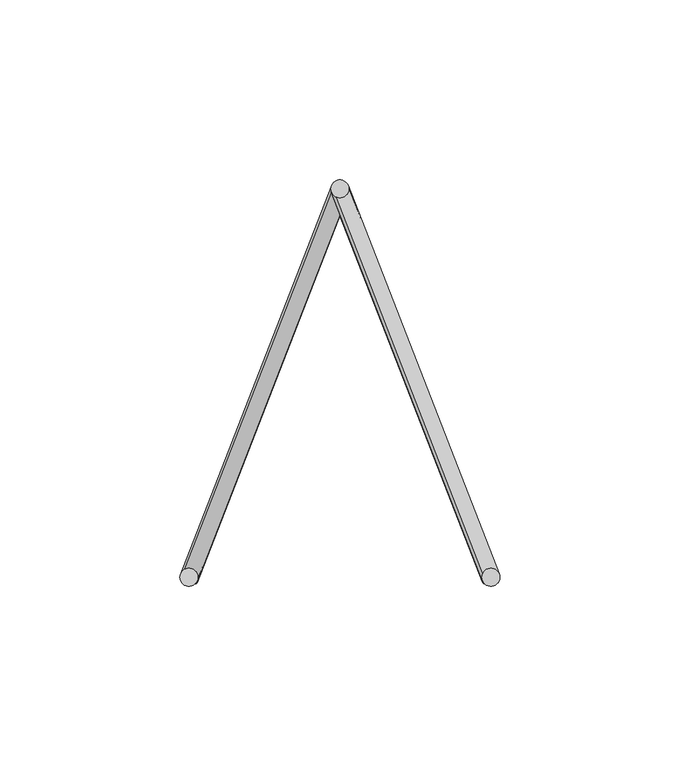
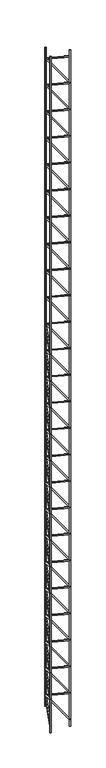
"""IFC4 building model written with IfcOpenShell, lengths in millimetres: proxy geometry, Pre-fab. (Vigota 7 - Pano 3)."""

import ifcopenshell
import ifcopenshell.guid

model = None  # the IFC model being written
_history = None  # IfcOwnerHistory: only IFC2X3 demands one
_inside = {}  # id of a spatial element -> (the spatial element, [elements in it])
_under = {}  # id of a project, library or spatial element -> (it, [spatial elements below it])
_declared = {}  # id of a project -> (the project, [libraries it declares])
_typed = {}  # id of a type object -> (the type object, [elements of that type])
_made_of = {}  # id of a material, layer set ... -> (it, [elements and type objects made of it])


def new_model(schema):
    """Start an empty IFC model of exactly this schema.

    Asked for "IFC4X3", IfcOpenShell would pick the latest addendum, in which some entities
    have other attributes; the version numbers below select the first issue.
    IFC2X3 requires an IfcOwnerHistory on every rooted entity: one is made here for all.
    """
    global model, _history
    if schema == "IFC4X3":
        model = ifcopenshell.file(schema_version=(4, 3, 0, 0))
    else:
        model = ifcopenshell.file(schema=schema)
    _inside.clear()
    _under.clear()
    _declared.clear()
    _typed.clear()
    _made_of.clear()
    _history = None
    if model.schema == "IFC2X3":
        org = make("IfcOrganization", Name="unknown")
        user = make(
            "IfcPersonAndOrganization",
            ThePerson=make("IfcPerson", FamilyName="unknown"),
            TheOrganization=org,
        )
        app = make(
            "IfcApplication",
            ApplicationDeveloper=org,
            Version="unknown",
            ApplicationFullName="unknown",
            ApplicationIdentifier="unknown",
        )
        _history = make(
            "IfcOwnerHistory",
            OwningUser=user,
            OwningApplication=app,
            ChangeAction="ADDED",
            CreationDate=0,
        )
    return model


def make(cls, **values):
    """One entity of the class cls with the attributes given. An attribute that is None is left unset."""
    return model.create_entity(
        cls, **{name: value for name, value in values.items() if value is not None}
    )


def rooted(cls, **values):
    """An entity with a GlobalId (a new one), such as an element, a storey or a relation."""
    return make(cls, GlobalId=ifcopenshell.guid.new(), OwnerHistory=_history, **values)


def si_unit(unit_type, name, prefix=None):
    """IfcSIUnit, for example si_unit("LENGTHUNIT", "METRE", prefix="MILLI")."""
    return make("IfcSIUnit", UnitType=unit_type, Prefix=prefix, Name=name)


def assignment(units):
    """IfcUnitAssignment: the units of a project."""
    return None if units is None else make("IfcUnitAssignment", Units=units)


def point(xyz):
    """IfcCartesianPoint."""
    return None if xyz is None else make("IfcCartesianPoint", Coordinates=xyz)


def direction(xyz):
    """IfcDirection."""
    return None if xyz is None else make("IfcDirection", DirectionRatios=xyz)


def frame(location, z_axis=None, x_axis=None):
    """IfcAxis2Placement3D, a coordinate frame: its origin and axes. An axis left out is left unset."""
    return make(
        "IfcAxis2Placement3D",
        Location=point(location),
        Axis=direction(z_axis),
        RefDirection=direction(x_axis),
    )


def frame_2d(location, x_axis=None):
    """IfcAxis2Placement2D, a coordinate frame in the plane: its origin and x axis."""
    return make(
        "IfcAxis2Placement2D", Location=point(location), RefDirection=direction(x_axis)
    )


def origin():
    """The frame at (0, 0, 0) with its axes left unset."""
    return frame((0.0, 0.0, 0.0))


def origin_with_axes():
    """The frame at (0, 0, 0) with the z axis (0, 0, 1) and the x axis (1, 0, 0) written out."""
    return frame((0.0, 0.0, 0.0), z_axis=(0.0, 0.0, 1.0), x_axis=(1.0, 0.0, 0.0))


def origin_2d():
    """The frame at (0, 0) in the plane with its x axis left unset."""
    return frame_2d((0.0, 0.0))


def place(relative_to, where):
    """IfcLocalPlacement: puts the frame where relative to a parent placement (None: the world)."""
    return make(
        "IfcLocalPlacement", PlacementRelTo=relative_to, RelativePlacement=where
    )


def context(
    kind, dimensions, precision=None, world=None, true_north=None, identifier=None
):
    """IfcGeometricRepresentationContext, for example the 3D "Model" context."""
    return make(
        "IfcGeometricRepresentationContext",
        ContextIdentifier=identifier,
        ContextType=kind,
        CoordinateSpaceDimension=dimensions,
        Precision=precision,
        WorldCoordinateSystem=world,
        TrueNorth=true_north,
    )


def project(units=None, contexts=None):
    """IfcProject with its units and contexts."""
    return rooted(
        "IfcProject",
        Name="project",
        RepresentationContexts=contexts,
        UnitsInContext=assignment(units),
    )


def spatial(cls, under=None, at=None, **own):
    """A site, building, storey or space (cls), placed at a placement, below another one or the project."""
    s = rooted(cls, ObjectPlacement=at, **own)
    if under is not None:
        _under.setdefault(under.id(), (under, []))[1].append(s)
    return s


def circle_curve(where, radius):
    """IfcCircle in the frame where."""
    return make("IfcCircle", Position=where, Radius=radius)


def trimmed(basis, trim1, trim2, sense, master):
    """IfcTrimmedCurve: the piece of a basis curve between two trims."""
    return make(
        "IfcTrimmedCurve",
        BasisCurve=basis,
        Trim1=trim1,
        Trim2=trim2,
        SenseAgreement=sense,
        MasterRepresentation=master,
    )


def segment(curve, same_sense, transition):
    """IfcCompositeCurveSegment."""
    return make(
        "IfcCompositeCurveSegment",
        Transition=transition,
        SameSense=same_sense,
        ParentCurve=curve,
    )


def composite_curve(segments, self_intersect=None):
    """IfcCompositeCurve: segments joined end to end."""
    return make("IfcCompositeCurve", Segments=segments, SelfIntersect=self_intersect)


def outline(outer, holes=None, kind="AREA"):
    """IfcArbitraryClosedProfileDef: a profile drawn as a closed curve; with holes, ...WithVoids."""
    if holes is None:
        return make("IfcArbitraryClosedProfileDef", ProfileType=kind, OuterCurve=outer)
    return make(
        "IfcArbitraryProfileDefWithVoids",
        ProfileType=kind,
        OuterCurve=outer,
        InnerCurves=holes,
    )


def extrude(swept, where, along, depth):
    """IfcExtrudedAreaSolid: the profile swept, set in the frame where, extruded along a direction by depth."""
    return make(
        "IfcExtrudedAreaSolid",
        SweptArea=swept,
        Position=where,
        ExtrudedDirection=direction(along),
        Depth=depth,
    )


def shape(context_of_items, identifier, shape_type, items):
    """IfcShapeRepresentation: the items that make up one representation, for example the "Body"."""
    return make(
        "IfcShapeRepresentation",
        ContextOfItems=context_of_items,
        RepresentationIdentifier=identifier,
        RepresentationType=shape_type,
        Items=items,
    )


def source(mapping_origin, context_of_items, identifier, shape_type, items):
    """IfcRepresentationMap: a shape defined once, which mapped items show again and again."""
    return make(
        "IfcRepresentationMap",
        MappingOrigin=mapping_origin,
        MappedRepresentation=shape(context_of_items, identifier, shape_type, items),
    )


def transform(
    local_origin,
    x_axis=None,
    y_axis=None,
    z_axis=None,
    scale=None,
    scale2=None,
    scale3=None,
    uniform=True,
):
    """IfcCartesianTransformationOperator3D, or its non-uniform kind. x_axis, y_axis, z_axis: its Axis1, 2, 3."""
    if uniform:
        return make(
            "IfcCartesianTransformationOperator3D",
            Axis1=direction(x_axis),
            Axis2=direction(y_axis),
            LocalOrigin=point(local_origin),
            Scale=scale,
            Axis3=direction(z_axis),
        )
    return make(
        "IfcCartesianTransformationOperator3DnonUniform",
        Axis1=direction(x_axis),
        Axis2=direction(y_axis),
        LocalOrigin=point(local_origin),
        Scale=scale,
        Axis3=direction(z_axis),
        Scale2=scale2,
        Scale3=scale3,
    )


def mapped(mapping_source, mapping_target):
    """IfcMappedItem: shows the shape of a source again, moved by a transform."""
    return make(
        "IfcMappedItem", MappingSource=mapping_source, MappingTarget=mapping_target
    )


def made_of(thing, what):
    """Note that an element or type object is made of a material, layer set ...; save() writes the relation."""
    if what is not None:
        _made_of.setdefault(what.id(), (what, []))[1].append(thing)
    return thing


def element(
    cls,
    number,
    at=None,
    inside=None,
    cuts=None,
    type_object=None,
    material=None,
    context=None,
    identifier="Body",
    shape_type=None,
    held_by="IfcProductDefinitionShape",
    body=None,
    shapes=None,
    **own,
):
    """One element of the class cls, such as IfcWall. Its Tag is "e" and its number.

    at: its placement. inside: the storey or other place that contains it. cuts: it is an
    opening in that element (IfcRelVoidsElement). A single representation is given by context,
    identifier, shape_type and body (its items); several are given by shapes. held_by: the class
    of the entity that holds the representations. save() writes the other relations.
    """
    e = rooted(cls, Tag="e%d" % number, ObjectPlacement=at, **own)
    if body is not None:
        shapes = [shape(context, identifier, shape_type, body)]
    if shapes is not None:
        e.Representation = make(held_by, Representations=shapes)
    if inside is not None:
        _inside.setdefault(inside.id(), (inside, []))[1].append(e)
    if cuts is not None:
        rooted(
            "IfcRelVoidsElement", RelatingBuildingElement=cuts, RelatedOpeningElement=e
        )
    if type_object is not None:
        _typed.setdefault(type_object.id(), (type_object, []))[1].append(e)
    return made_of(e, material)


def aggregate(whole, parts):
    """IfcRelAggregates: a whole, such as a stair, and the parts it consists of."""
    return rooted("IfcRelAggregates", RelatingObject=whole, RelatedObjects=parts)


def save(model, path):
    """Write the relations noted so far, then the file.

    IfcRelAggregates (storeys below a building ...), IfcRelContainedInSpatialStructure (elements
    in a storey), IfcRelDefinesByType, IfcRelAssociatesMaterial and IfcRelDeclares: one each for
    every whole, place, type object, material and project.
    """
    for whole, parts in _under.values():
        aggregate(whole, parts)
    for where, things in _inside.values():
        rooted(
            "IfcRelContainedInSpatialStructure",
            RelatedElements=things,
            RelatingStructure=where,
        )
    for kind, things in _typed.values():
        rooted("IfcRelDefinesByType", RelatedObjects=things, RelatingType=kind)
    for what, things in _made_of.values():
        rooted("IfcRelAssociatesMaterial", RelatedObjects=things, RelatingMaterial=what)
    for by, libraries in _declared.values():
        rooted("IfcRelDeclares", RelatingContext=by, RelatedDefinitions=libraries)
    model.write(path)


def structural_framing_d1675b47(model_context):
    return source(origin(), model_context, "Body", "SweptSolid", [
        extrude(outline(composite_curve([segment(trimmed(circle_curve(origin_2d(), 2.5), [point((2.5, 0.0))], [point((-2.5, 0.0))], False, "CARTESIAN"), True, "CONTINUOUS"), segment(trimmed(circle_curve(origin_2d(), 2.5), [point((-2.5, 0.0))], [point((2.5, 0.0))], False, "CARTESIAN"), True, "CONTINUOUS")], self_intersect=False)), origin_with_axes(), (0.0, 0.0, 1.0), 3059.00107),
        extrude(outline(composite_curve([segment(trimmed(circle_curve(frame_2d((-42.0, 108.0)), 2.5), [point((-39.5, 108.0))], [point((-44.5, 108.0))], False, "CARTESIAN"), True, "CONTINUOUS"), segment(trimmed(circle_curve(frame_2d((-42.0, 108.0)), 2.5), [point((-44.5, 108.0))], [point((-39.5, 108.0))], False, "CARTESIAN"), True, "CONTINUOUS")], self_intersect=False)), frame((0.0, 0.0, 39.500535), z_axis=(0.0, 0.0, 1.0), x_axis=(1.0, 0.0, 0.0)), (0.0, 0.0, 1.0), 2980.0),
        extrude(outline(composite_curve([segment(trimmed(circle_curve(origin_2d(), 2.5), [point((2.5, 0.0))], [point((-2.5, 0.0))], False, "CARTESIAN"), True, "CONTINUOUS"), segment(trimmed(circle_curve(origin_2d(), 2.5), [point((-2.5, 0.0))], [point((2.5, 0.0))], False, "CARTESIAN"), True, "CONTINUOUS")], self_intersect=False)), frame((0.0, 0.0, 29.500535), z_axis=(-0.3218603428886276, 0.8276408817707567, 0.4598004898837537), x_axis=(0.8192319205108605, -3.936835275445103e-11, 0.5734623443750141)), (0.0, 0.0, 1.0), 130.491379),
        extrude(outline(composite_curve([segment(trimmed(circle_curve(origin_2d(), 2.5), [point((2.5, 0.0))], [point((-2.5, 0.0))], False, "CARTESIAN"), True, "CONTINUOUS"), segment(trimmed(circle_curve(origin_2d(), 2.5), [point((-2.5, 0.0))], [point((2.5, 0.0))], False, "CARTESIAN"), True, "CONTINUOUS")], self_intersect=False)), frame((-42.0, 108.0, 89.500535), z_axis=(0.3218603428886276, -0.8276408817707567, 0.4598004898837537), x_axis=(0.8192319205108605, -3.936835275445103e-11, -0.5734623443750141)), (0.0, 0.0, 1.0), 130.491379),
        extrude(outline(composite_curve([segment(trimmed(circle_curve(origin_2d(), 2.5), [point((2.5, 0.0))], [point((-2.5, 0.0))], False, "CARTESIAN"), True, "CONTINUOUS"), segment(trimmed(circle_curve(origin_2d(), 2.5), [point((-2.5, 0.0))], [point((2.5, 0.0))], False, "CARTESIAN"), True, "CONTINUOUS")], self_intersect=False)), frame((0.0, 0.0, 149.500535), z_axis=(-0.3218603428886276, 0.8276408817707567, 0.4598004898837537), x_axis=(0.8192319205108605, -3.936835275445103e-11, 0.5734623443750141)), (0.0, 0.0, 1.0), 130.491379),
        extrude(outline(composite_curve([segment(trimmed(circle_curve(origin_2d(), 2.5), [point((2.5, 0.0))], [point((-2.5, 0.0))], False, "CARTESIAN"), True, "CONTINUOUS"), segment(trimmed(circle_curve(origin_2d(), 2.5), [point((-2.5, 0.0))], [point((2.5, 0.0))], False, "CARTESIAN"), True, "CONTINUOUS")], self_intersect=False)), frame((-42.0, 108.0, 209.500535), z_axis=(0.3218603428886276, -0.8276408817707567, 0.4598004898837537), x_axis=(0.8192319205108605, -3.936835275445103e-11, -0.5734623443750141)), (0.0, 0.0, 1.0), 130.491379),
        extrude(outline(composite_curve([segment(trimmed(circle_curve(origin_2d(), 2.5), [point((2.5, 0.0))], [point((-2.5, 0.0))], False, "CARTESIAN"), True, "CONTINUOUS"), segment(trimmed(circle_curve(origin_2d(), 2.5), [point((-2.5, 0.0))], [point((2.5, 0.0))], False, "CARTESIAN"), True, "CONTINUOUS")], self_intersect=False)), frame((0.0, 0.0, 269.500535), z_axis=(-0.3218603428886276, 0.8276408817707567, 0.4598004898837537), x_axis=(0.8192319205108605, -3.936835275445103e-11, 0.5734623443750141)), (0.0, 0.0, 1.0), 130.491379),
        extrude(outline(composite_curve([segment(trimmed(circle_curve(origin_2d(), 2.5), [point((2.5, 0.0))], [point((-2.5, 0.0))], False, "CARTESIAN"), True, "CONTINUOUS"), segment(trimmed(circle_curve(origin_2d(), 2.5), [point((-2.5, 0.0))], [point((2.5, 0.0))], False, "CARTESIAN"), True, "CONTINUOUS")], self_intersect=False)), frame((-42.0, 108.0, 329.500535), z_axis=(0.3218603428886276, -0.8276408817707567, 0.4598004898837537), x_axis=(0.8192319205108605, -3.936835275445103e-11, -0.5734623443750141)), (0.0, 0.0, 1.0), 130.491379),
        extrude(outline(composite_curve([segment(trimmed(circle_curve(origin_2d(), 2.5), [point((2.5, 0.0))], [point((-2.5, 0.0))], False, "CARTESIAN"), True, "CONTINUOUS"), segment(trimmed(circle_curve(origin_2d(), 2.5), [point((-2.5, 0.0))], [point((2.5, 0.0))], False, "CARTESIAN"), True, "CONTINUOUS")], self_intersect=False)), frame((0.0, 0.0, 389.500535), z_axis=(-0.3218603428886276, 0.8276408817707567, 0.4598004898837537), x_axis=(0.8192319205108605, -3.936835275445103e-11, 0.5734623443750141)), (0.0, 0.0, 1.0), 130.491379),
        extrude(outline(composite_curve([segment(trimmed(circle_curve(origin_2d(), 2.5), [point((2.5, 0.0))], [point((-2.5, 0.0))], False, "CARTESIAN"), True, "CONTINUOUS"), segment(trimmed(circle_curve(origin_2d(), 2.5), [point((-2.5, 0.0))], [point((2.5, 0.0))], False, "CARTESIAN"), True, "CONTINUOUS")], self_intersect=False)), frame((-42.0, 108.0, 449.500535), z_axis=(0.3218603428886276, -0.8276408817707567, 0.4598004898837537), x_axis=(0.8192319205108605, -3.936835275445103e-11, -0.5734623443750141)), (0.0, 0.0, 1.0), 130.491379),
        extrude(outline(composite_curve([segment(trimmed(circle_curve(origin_2d(), 2.5), [point((2.5, 0.0))], [point((-2.5, 0.0))], False, "CARTESIAN"), True, "CONTINUOUS"), segment(trimmed(circle_curve(origin_2d(), 2.5), [point((-2.5, 0.0))], [point((2.5, 0.0))], False, "CARTESIAN"), True, "CONTINUOUS")], self_intersect=False)), frame((0.0, 0.0, 509.500535), z_axis=(-0.3218603428886276, 0.8276408817707567, 0.4598004898837537), x_axis=(0.8192319205108605, -3.936835275445103e-11, 0.5734623443750141)), (0.0, 0.0, 1.0), 130.491379),
        extrude(outline(composite_curve([segment(trimmed(circle_curve(origin_2d(), 2.5), [point((2.5, 0.0))], [point((-2.5, 0.0))], False, "CARTESIAN"), True, "CONTINUOUS"), segment(trimmed(circle_curve(origin_2d(), 2.5), [point((-2.5, 0.0))], [point((2.5, 0.0))], False, "CARTESIAN"), True, "CONTINUOUS")], self_intersect=False)), frame((-42.0, 108.0, 569.500535), z_axis=(0.3218603428886276, -0.8276408817707567, 0.4598004898837537), x_axis=(0.8192319205108605, -3.936835275445103e-11, -0.5734623443750141)), (0.0, 0.0, 1.0), 130.491379),
        extrude(outline(composite_curve([segment(trimmed(circle_curve(origin_2d(), 2.5), [point((2.5, 0.0))], [point((-2.5, 0.0))], False, "CARTESIAN"), True, "CONTINUOUS"), segment(trimmed(circle_curve(origin_2d(), 2.5), [point((-2.5, 0.0))], [point((2.5, 0.0))], False, "CARTESIAN"), True, "CONTINUOUS")], self_intersect=False)), frame((0.0, 0.0, 629.500535), z_axis=(-0.3218603428886276, 0.8276408817707567, 0.4598004898837537), x_axis=(0.8192319205108605, -3.936835275445103e-11, 0.5734623443750141)), (0.0, 0.0, 1.0), 130.491379),
        extrude(outline(composite_curve([segment(trimmed(circle_curve(origin_2d(), 2.5), [point((2.5, 0.0))], [point((-2.5, 0.0))], False, "CARTESIAN"), True, "CONTINUOUS"), segment(trimmed(circle_curve(origin_2d(), 2.5), [point((-2.5, 0.0))], [point((2.5, 0.0))], False, "CARTESIAN"), True, "CONTINUOUS")], self_intersect=False)), frame((-42.0, 108.0, 689.500535), z_axis=(0.3218603428886276, -0.8276408817707567, 0.4598004898837537), x_axis=(0.8192319205108605, -3.936835275445103e-11, -0.5734623443750141)), (0.0, 0.0, 1.0), 130.491379),
        extrude(outline(composite_curve([segment(trimmed(circle_curve(origin_2d(), 2.5), [point((2.5, 0.0))], [point((-2.5, 0.0))], False, "CARTESIAN"), True, "CONTINUOUS"), segment(trimmed(circle_curve(origin_2d(), 2.5), [point((-2.5, 0.0))], [point((2.5, 0.0))], False, "CARTESIAN"), True, "CONTINUOUS")], self_intersect=False)), frame((0.0, 0.0, 749.500535), z_axis=(-0.3218603428886276, 0.8276408817707567, 0.4598004898837537), x_axis=(0.8192319205108605, -3.936835275445103e-11, 0.5734623443750141)), (0.0, 0.0, 1.0), 130.491379),
        extrude(outline(composite_curve([segment(trimmed(circle_curve(origin_2d(), 2.5), [point((2.5, 0.0))], [point((-2.5, 0.0))], False, "CARTESIAN"), True, "CONTINUOUS"), segment(trimmed(circle_curve(origin_2d(), 2.5), [point((-2.5, 0.0))], [point((2.5, 0.0))], False, "CARTESIAN"), True, "CONTINUOUS")], self_intersect=False)), frame((-42.0, 108.0, 809.500535), z_axis=(0.3218603428886276, -0.8276408817707567, 0.4598004898837537), x_axis=(0.8192319205108605, -3.936835275445103e-11, -0.5734623443750141)), (0.0, 0.0, 1.0), 130.491379),
        extrude(outline(composite_curve([segment(trimmed(circle_curve(origin_2d(), 2.5), [point((2.5, 0.0))], [point((-2.5, 0.0))], False, "CARTESIAN"), True, "CONTINUOUS"), segment(trimmed(circle_curve(origin_2d(), 2.5), [point((-2.5, 0.0))], [point((2.5, 0.0))], False, "CARTESIAN"), True, "CONTINUOUS")], self_intersect=False)), frame((0.0, 0.0, 869.500535), z_axis=(-0.3218603428886276, 0.8276408817707567, 0.4598004898837537), x_axis=(0.8192319205108605, -3.936835275445103e-11, 0.5734623443750141)), (0.0, 0.0, 1.0), 130.491379),
        extrude(outline(composite_curve([segment(trimmed(circle_curve(origin_2d(), 2.5), [point((2.5, 0.0))], [point((-2.5, 0.0))], False, "CARTESIAN"), True, "CONTINUOUS"), segment(trimmed(circle_curve(origin_2d(), 2.5), [point((-2.5, 0.0))], [point((2.5, 0.0))], False, "CARTESIAN"), True, "CONTINUOUS")], self_intersect=False)), frame((-42.0, 108.0, 929.500535), z_axis=(0.3218603428886276, -0.8276408817707567, 0.4598004898837537), x_axis=(0.8192319205108605, -3.936835275445103e-11, -0.5734623443750141)), (0.0, 0.0, 1.0), 130.491379),
        extrude(outline(composite_curve([segment(trimmed(circle_curve(origin_2d(), 2.5), [point((2.5, 0.0))], [point((-2.5, 0.0))], False, "CARTESIAN"), True, "CONTINUOUS"), segment(trimmed(circle_curve(origin_2d(), 2.5), [point((-2.5, 0.0))], [point((2.5, 0.0))], False, "CARTESIAN"), True, "CONTINUOUS")], self_intersect=False)), frame((0.0, 0.0, 989.500535), z_axis=(-0.3218603428886276, 0.8276408817707567, 0.4598004898837537), x_axis=(0.8192319205108605, -3.936835275445103e-11, 0.5734623443750141)), (0.0, 0.0, 1.0), 130.491379),
        extrude(outline(composite_curve([segment(trimmed(circle_curve(origin_2d(), 2.5), [point((2.5, 0.0))], [point((-2.5, 0.0))], False, "CARTESIAN"), True, "CONTINUOUS"), segment(trimmed(circle_curve(origin_2d(), 2.5), [point((-2.5, 0.0))], [point((2.5, 0.0))], False, "CARTESIAN"), True, "CONTINUOUS")], self_intersect=False)), frame((-42.0, 108.0, 1049.500535), z_axis=(0.3218603428886276, -0.8276408817707567, 0.4598004898837537), x_axis=(0.8192319205108605, -3.936835275445103e-11, -0.5734623443750141)), (0.0, 0.0, 1.0), 130.491379),
        extrude(outline(composite_curve([segment(trimmed(circle_curve(origin_2d(), 2.5), [point((2.5, 0.0))], [point((-2.5, 0.0))], False, "CARTESIAN"), True, "CONTINUOUS"), segment(trimmed(circle_curve(origin_2d(), 2.5), [point((-2.5, 0.0))], [point((2.5, 0.0))], False, "CARTESIAN"), True, "CONTINUOUS")], self_intersect=False)), frame((0.0, 0.0, 1109.500535), z_axis=(-0.3218603428886276, 0.8276408817707567, 0.4598004898837537), x_axis=(0.8192319205108605, -3.936835275445103e-11, 0.5734623443750141)), (0.0, 0.0, 1.0), 130.491379),
        extrude(outline(composite_curve([segment(trimmed(circle_curve(origin_2d(), 2.5), [point((2.5, 0.0))], [point((-2.5, 0.0))], False, "CARTESIAN"), True, "CONTINUOUS"), segment(trimmed(circle_curve(origin_2d(), 2.5), [point((-2.5, 0.0))], [point((2.5, 0.0))], False, "CARTESIAN"), True, "CONTINUOUS")], self_intersect=False)), frame((-42.0, 108.0, 1169.500535), z_axis=(0.3218603428886276, -0.8276408817707567, 0.4598004898837537), x_axis=(0.8192319205108605, -3.936835275445103e-11, -0.5734623443750141)), (0.0, 0.0, 1.0), 130.491379),
        extrude(outline(composite_curve([segment(trimmed(circle_curve(origin_2d(), 2.5), [point((2.5, 0.0))], [point((-2.5, 0.0))], False, "CARTESIAN"), True, "CONTINUOUS"), segment(trimmed(circle_curve(origin_2d(), 2.5), [point((-2.5, 0.0))], [point((2.5, 0.0))], False, "CARTESIAN"), True, "CONTINUOUS")], self_intersect=False)), frame((0.0, 0.0, 1229.500535), z_axis=(-0.3218603428886276, 0.8276408817707567, 0.4598004898837537), x_axis=(0.8192319205108605, -3.936835275445103e-11, 0.5734623443750141)), (0.0, 0.0, 1.0), 130.491379),
        extrude(outline(composite_curve([segment(trimmed(circle_curve(origin_2d(), 2.5), [point((2.5, 0.0))], [point((-2.5, 0.0))], False, "CARTESIAN"), True, "CONTINUOUS"), segment(trimmed(circle_curve(origin_2d(), 2.5), [point((-2.5, 0.0))], [point((2.5, 0.0))], False, "CARTESIAN"), True, "CONTINUOUS")], self_intersect=False)), frame((-42.0, 108.0, 1289.500535), z_axis=(0.3218603428886276, -0.8276408817707567, 0.4598004898837537), x_axis=(0.8192319205108605, -3.936835275445103e-11, -0.5734623443750141)), (0.0, 0.0, 1.0), 130.491379),
        extrude(outline(composite_curve([segment(trimmed(circle_curve(origin_2d(), 2.5), [point((2.5, 0.0))], [point((-2.5, 0.0))], False, "CARTESIAN"), True, "CONTINUOUS"), segment(trimmed(circle_curve(origin_2d(), 2.5), [point((-2.5, 0.0))], [point((2.5, 0.0))], False, "CARTESIAN"), True, "CONTINUOUS")], self_intersect=False)), frame((0.0, 0.0, 1349.500535), z_axis=(-0.3218603428886276, 0.8276408817707567, 0.4598004898837537), x_axis=(0.8192319205108605, -3.936835275445103e-11, 0.5734623443750141)), (0.0, 0.0, 1.0), 130.491379),
        extrude(outline(composite_curve([segment(trimmed(circle_curve(origin_2d(), 2.5), [point((2.5, 0.0))], [point((-2.5, 0.0))], False, "CARTESIAN"), True, "CONTINUOUS"), segment(trimmed(circle_curve(origin_2d(), 2.5), [point((-2.5, 0.0))], [point((2.5, 0.0))], False, "CARTESIAN"), True, "CONTINUOUS")], self_intersect=False)), frame((-42.0, 108.0, 1409.500535), z_axis=(0.3218603428886276, -0.8276408817707567, 0.4598004898837537), x_axis=(0.8192319205108605, -3.936835275445103e-11, -0.5734623443750141)), (0.0, 0.0, 1.0), 130.491379),
        extrude(outline(composite_curve([segment(trimmed(circle_curve(origin_2d(), 2.5), [point((2.5, 0.0))], [point((-2.5, 0.0))], False, "CARTESIAN"), True, "CONTINUOUS"), segment(trimmed(circle_curve(origin_2d(), 2.5), [point((-2.5, 0.0))], [point((2.5, 0.0))], False, "CARTESIAN"), True, "CONTINUOUS")], self_intersect=False)), frame((0.0, 0.0, 1469.500535), z_axis=(-0.3218603428886276, 0.8276408817707567, 0.4598004898837537), x_axis=(0.8192319205108605, -3.936835275445103e-11, 0.5734623443750141)), (0.0, 0.0, 1.0), 130.491379),
        extrude(outline(composite_curve([segment(trimmed(circle_curve(origin_2d(), 2.5), [point((2.5, 0.0))], [point((-2.5, 0.0))], False, "CARTESIAN"), True, "CONTINUOUS"), segment(trimmed(circle_curve(origin_2d(), 2.5), [point((-2.5, 0.0))], [point((2.5, 0.0))], False, "CARTESIAN"), True, "CONTINUOUS")], self_intersect=False)), frame((-42.0, 108.0, 1529.500535), z_axis=(0.3218603428886276, -0.8276408817707567, 0.4598004898837537), x_axis=(0.8192319205108605, -3.936835275445103e-11, -0.5734623443750141)), (0.0, 0.0, 1.0), 130.491379),
        extrude(outline(composite_curve([segment(trimmed(circle_curve(origin_2d(), 2.5), [point((2.5, 0.0))], [point((-2.5, 0.0))], False, "CARTESIAN"), True, "CONTINUOUS"), segment(trimmed(circle_curve(origin_2d(), 2.5), [point((-2.5, 0.0))], [point((2.5, 0.0))], False, "CARTESIAN"), True, "CONTINUOUS")], self_intersect=False)), frame((0.0, 0.0, 1589.500535), z_axis=(-0.3218603428886276, 0.8276408817707567, 0.4598004898837537), x_axis=(0.8192319205108605, -3.936835275445103e-11, 0.5734623443750141)), (0.0, 0.0, 1.0), 130.491379),
        extrude(outline(composite_curve([segment(trimmed(circle_curve(origin_2d(), 2.5), [point((2.5, 0.0))], [point((-2.5, 0.0))], False, "CARTESIAN"), True, "CONTINUOUS"), segment(trimmed(circle_curve(origin_2d(), 2.5), [point((-2.5, 0.0))], [point((2.5, 0.0))], False, "CARTESIAN"), True, "CONTINUOUS")], self_intersect=False)), frame((-42.0, 108.0, 1649.500535), z_axis=(0.3218603428886276, -0.8276408817707567, 0.4598004898837537), x_axis=(0.8192319205108605, -3.936835275445103e-11, -0.5734623443750141)), (0.0, 0.0, 1.0), 130.491379),
        extrude(outline(composite_curve([segment(trimmed(circle_curve(origin_2d(), 2.5), [point((2.5, 0.0))], [point((-2.5, 0.0))], False, "CARTESIAN"), True, "CONTINUOUS"), segment(trimmed(circle_curve(origin_2d(), 2.5), [point((-2.5, 0.0))], [point((2.5, 0.0))], False, "CARTESIAN"), True, "CONTINUOUS")], self_intersect=False)), frame((0.0, 0.0, 1709.500535), z_axis=(-0.3218603428886276, 0.8276408817707567, 0.4598004898837537), x_axis=(0.8192319205108605, -3.936835275445103e-11, 0.5734623443750141)), (0.0, 0.0, 1.0), 130.491379),
        extrude(outline(composite_curve([segment(trimmed(circle_curve(origin_2d(), 2.5), [point((2.5, 0.0))], [point((-2.5, 0.0))], False, "CARTESIAN"), True, "CONTINUOUS"), segment(trimmed(circle_curve(origin_2d(), 2.5), [point((-2.5, 0.0))], [point((2.5, 0.0))], False, "CARTESIAN"), True, "CONTINUOUS")], self_intersect=False)), frame((-42.0, 108.0, 1769.500535), z_axis=(0.3218603428886276, -0.8276408817707567, 0.4598004898837537), x_axis=(0.8192319205108605, -3.936835275445103e-11, -0.5734623443750141)), (0.0, 0.0, 1.0), 130.491379),
        extrude(outline(composite_curve([segment(trimmed(circle_curve(origin_2d(), 2.5), [point((2.5, 0.0))], [point((-2.5, 0.0))], False, "CARTESIAN"), True, "CONTINUOUS"), segment(trimmed(circle_curve(origin_2d(), 2.5), [point((-2.5, 0.0))], [point((2.5, 0.0))], False, "CARTESIAN"), True, "CONTINUOUS")], self_intersect=False)), frame((0.0, 0.0, 1829.500535), z_axis=(-0.3218603428886276, 0.8276408817707567, 0.4598004898837537), x_axis=(0.8192319205108605, -3.936835275445103e-11, 0.5734623443750141)), (0.0, 0.0, 1.0), 130.491379),
        extrude(outline(composite_curve([segment(trimmed(circle_curve(origin_2d(), 2.5), [point((2.5, 0.0))], [point((-2.5, 0.0))], False, "CARTESIAN"), True, "CONTINUOUS"), segment(trimmed(circle_curve(origin_2d(), 2.5), [point((-2.5, 0.0))], [point((2.5, 0.0))], False, "CARTESIAN"), True, "CONTINUOUS")], self_intersect=False)), frame((-42.0, 108.0, 1889.500535), z_axis=(0.3218603428886276, -0.8276408817707567, 0.4598004898837537), x_axis=(0.8192319205108605, -3.936835275445103e-11, -0.5734623443750141)), (0.0, 0.0, 1.0), 130.491379),
        extrude(outline(composite_curve([segment(trimmed(circle_curve(origin_2d(), 2.5), [point((2.5, 0.0))], [point((-2.5, 0.0))], False, "CARTESIAN"), True, "CONTINUOUS"), segment(trimmed(circle_curve(origin_2d(), 2.5), [point((-2.5, 0.0))], [point((2.5, 0.0))], False, "CARTESIAN"), True, "CONTINUOUS")], self_intersect=False)), frame((0.0, 0.0, 1949.500535), z_axis=(-0.3218603428886276, 0.8276408817707567, 0.4598004898837537), x_axis=(0.8192319205108605, -3.936835275445103e-11, 0.5734623443750141)), (0.0, 0.0, 1.0), 130.491379),
        extrude(outline(composite_curve([segment(trimmed(circle_curve(origin_2d(), 2.5), [point((2.5, 0.0))], [point((-2.5, 0.0))], False, "CARTESIAN"), True, "CONTINUOUS"), segment(trimmed(circle_curve(origin_2d(), 2.5), [point((-2.5, 0.0))], [point((2.5, 0.0))], False, "CARTESIAN"), True, "CONTINUOUS")], self_intersect=False)), frame((-42.0, 108.0, 2009.500535), z_axis=(0.3218603428886276, -0.8276408817707567, 0.4598004898837537), x_axis=(0.8192319205108605, -3.936835275445103e-11, -0.5734623443750141)), (0.0, 0.0, 1.0), 130.491379),
        extrude(outline(composite_curve([segment(trimmed(circle_curve(origin_2d(), 2.5), [point((2.5, 0.0))], [point((-2.5, 0.0))], False, "CARTESIAN"), True, "CONTINUOUS"), segment(trimmed(circle_curve(origin_2d(), 2.5), [point((-2.5, 0.0))], [point((2.5, 0.0))], False, "CARTESIAN"), True, "CONTINUOUS")], self_intersect=False)), frame((0.0, 0.0, 2069.500535), z_axis=(-0.3218603428886276, 0.8276408817707567, 0.4598004898837537), x_axis=(0.8192319205108605, -3.936835275445103e-11, 0.5734623443750141)), (0.0, 0.0, 1.0), 130.491379),
        extrude(outline(composite_curve([segment(trimmed(circle_curve(origin_2d(), 2.5), [point((2.5, 0.0))], [point((-2.5, 0.0))], False, "CARTESIAN"), True, "CONTINUOUS"), segment(trimmed(circle_curve(origin_2d(), 2.5), [point((-2.5, 0.0))], [point((2.5, 0.0))], False, "CARTESIAN"), True, "CONTINUOUS")], self_intersect=False)), frame((-42.0, 108.0, 2129.500535), z_axis=(0.3218603428886276, -0.8276408817707567, 0.4598004898837537), x_axis=(0.8192319205108605, -3.936835275445103e-11, -0.5734623443750141)), (0.0, 0.0, 1.0), 130.491379),
        extrude(outline(composite_curve([segment(trimmed(circle_curve(origin_2d(), 2.5), [point((2.5, 0.0))], [point((-2.5, 0.0))], False, "CARTESIAN"), True, "CONTINUOUS"), segment(trimmed(circle_curve(origin_2d(), 2.5), [point((-2.5, 0.0))], [point((2.5, 0.0))], False, "CARTESIAN"), True, "CONTINUOUS")], self_intersect=False)), frame((0.0, 0.0, 2189.500535), z_axis=(-0.3218603428886276, 0.8276408817707567, 0.4598004898837537), x_axis=(0.8192319205108605, -3.936835275445103e-11, 0.5734623443750141)), (0.0, 0.0, 1.0), 130.491379),
        extrude(outline(composite_curve([segment(trimmed(circle_curve(origin_2d(), 2.5), [point((2.5, 0.0))], [point((-2.5, 0.0))], False, "CARTESIAN"), True, "CONTINUOUS"), segment(trimmed(circle_curve(origin_2d(), 2.5), [point((-2.5, 0.0))], [point((2.5, 0.0))], False, "CARTESIAN"), True, "CONTINUOUS")], self_intersect=False)), frame((-42.0, 108.0, 2249.500535), z_axis=(0.3218603428886276, -0.8276408817707567, 0.4598004898837537), x_axis=(0.8192319205108605, -3.936835275445103e-11, -0.5734623443750141)), (0.0, 0.0, 1.0), 130.491379),
        extrude(outline(composite_curve([segment(trimmed(circle_curve(origin_2d(), 2.5), [point((2.5, 0.0))], [point((-2.5, 0.0))], False, "CARTESIAN"), True, "CONTINUOUS"), segment(trimmed(circle_curve(origin_2d(), 2.5), [point((-2.5, 0.0))], [point((2.5, 0.0))], False, "CARTESIAN"), True, "CONTINUOUS")], self_intersect=False)), frame((0.0, 0.0, 2309.500535), z_axis=(-0.3218603428886276, 0.8276408817707567, 0.4598004898837537), x_axis=(0.8192319205108605, -3.936835275445103e-11, 0.5734623443750141)), (0.0, 0.0, 1.0), 130.491379),
        extrude(outline(composite_curve([segment(trimmed(circle_curve(origin_2d(), 2.5), [point((2.5, 0.0))], [point((-2.5, 0.0))], False, "CARTESIAN"), True, "CONTINUOUS"), segment(trimmed(circle_curve(origin_2d(), 2.5), [point((-2.5, 0.0))], [point((2.5, 0.0))], False, "CARTESIAN"), True, "CONTINUOUS")], self_intersect=False)), frame((-42.0, 108.0, 2369.500535), z_axis=(0.3218603428886276, -0.8276408817707567, 0.4598004898837537), x_axis=(0.8192319205108605, -3.936835275445103e-11, -0.5734623443750141)), (0.0, 0.0, 1.0), 130.491379),
        extrude(outline(composite_curve([segment(trimmed(circle_curve(origin_2d(), 2.5), [point((2.5, 0.0))], [point((-2.5, 0.0))], False, "CARTESIAN"), True, "CONTINUOUS"), segment(trimmed(circle_curve(origin_2d(), 2.5), [point((-2.5, 0.0))], [point((2.5, 0.0))], False, "CARTESIAN"), True, "CONTINUOUS")], self_intersect=False)), frame((0.0, 0.0, 2429.500535), z_axis=(-0.3218603428886276, 0.8276408817707567, 0.4598004898837537), x_axis=(0.8192319205108605, -3.936835275445103e-11, 0.5734623443750141)), (0.0, 0.0, 1.0), 130.491379),
        extrude(outline(composite_curve([segment(trimmed(circle_curve(origin_2d(), 2.5), [point((2.5, 0.0))], [point((-2.5, 0.0))], False, "CARTESIAN"), True, "CONTINUOUS"), segment(trimmed(circle_curve(origin_2d(), 2.5), [point((-2.5, 0.0))], [point((2.5, 0.0))], False, "CARTESIAN"), True, "CONTINUOUS")], self_intersect=False)), frame((-42.0, 108.0, 2489.500535), z_axis=(0.3218603428886276, -0.8276408817707567, 0.4598004898837537), x_axis=(0.8192319205108605, -3.936835275445103e-11, -0.5734623443750141)), (0.0, 0.0, 1.0), 130.491379),
        extrude(outline(composite_curve([segment(trimmed(circle_curve(origin_2d(), 2.5), [point((2.5, 0.0))], [point((-2.5, 0.0))], False, "CARTESIAN"), True, "CONTINUOUS"), segment(trimmed(circle_curve(origin_2d(), 2.5), [point((-2.5, 0.0))], [point((2.5, 0.0))], False, "CARTESIAN"), True, "CONTINUOUS")], self_intersect=False)), frame((0.0, 0.0, 2549.500535), z_axis=(-0.3218603428886276, 0.8276408817707567, 0.4598004898837537), x_axis=(0.8192319205108605, -3.936835275445103e-11, 0.5734623443750141)), (0.0, 0.0, 1.0), 130.491379),
        extrude(outline(composite_curve([segment(trimmed(circle_curve(origin_2d(), 2.5), [point((2.5, 0.0))], [point((-2.5, 0.0))], False, "CARTESIAN"), True, "CONTINUOUS"), segment(trimmed(circle_curve(origin_2d(), 2.5), [point((-2.5, 0.0))], [point((2.5, 0.0))], False, "CARTESIAN"), True, "CONTINUOUS")], self_intersect=False)), frame((-42.0, 108.0, 2609.500535), z_axis=(0.3218603428886276, -0.8276408817707567, 0.4598004898837537), x_axis=(0.8192319205108605, -3.936835275445103e-11, -0.5734623443750141)), (0.0, 0.0, 1.0), 130.491379),
        extrude(outline(composite_curve([segment(trimmed(circle_curve(origin_2d(), 2.5), [point((2.5, 0.0))], [point((-2.5, 0.0))], False, "CARTESIAN"), True, "CONTINUOUS"), segment(trimmed(circle_curve(origin_2d(), 2.5), [point((-2.5, 0.0))], [point((2.5, 0.0))], False, "CARTESIAN"), True, "CONTINUOUS")], self_intersect=False)), frame((0.0, 0.0, 2669.500535), z_axis=(-0.3218603428886276, 0.8276408817707567, 0.4598004898837537), x_axis=(0.8192319205108605, -3.936835275445103e-11, 0.5734623443750141)), (0.0, 0.0, 1.0), 130.491379),
        extrude(outline(composite_curve([segment(trimmed(circle_curve(origin_2d(), 2.5), [point((2.5, 0.0))], [point((-2.5, 0.0))], False, "CARTESIAN"), True, "CONTINUOUS"), segment(trimmed(circle_curve(origin_2d(), 2.5), [point((-2.5, 0.0))], [point((2.5, 0.0))], False, "CARTESIAN"), True, "CONTINUOUS")], self_intersect=False)), frame((-42.0, 108.0, 2729.500535), z_axis=(0.3218603428886276, -0.8276408817707567, 0.4598004898837537), x_axis=(0.8192319205108605, -3.936835275445103e-11, -0.5734623443750141)), (0.0, 0.0, 1.0), 130.491379),
        extrude(outline(composite_curve([segment(trimmed(circle_curve(origin_2d(), 2.5), [point((2.5, 0.0))], [point((-2.5, 0.0))], False, "CARTESIAN"), True, "CONTINUOUS"), segment(trimmed(circle_curve(origin_2d(), 2.5), [point((-2.5, 0.0))], [point((2.5, 0.0))], False, "CARTESIAN"), True, "CONTINUOUS")], self_intersect=False)), frame((0.0, 0.0, 2789.500535), z_axis=(-0.3218603428886276, 0.8276408817707567, 0.4598004898837537), x_axis=(0.8192319205108605, -3.936835275445103e-11, 0.5734623443750141)), (0.0, 0.0, 1.0), 130.491379),
        extrude(outline(composite_curve([segment(trimmed(circle_curve(origin_2d(), 2.5), [point((2.5, 0.0))], [point((-2.5, 0.0))], False, "CARTESIAN"), True, "CONTINUOUS"), segment(trimmed(circle_curve(origin_2d(), 2.5), [point((-2.5, 0.0))], [point((2.5, 0.0))], False, "CARTESIAN"), True, "CONTINUOUS")], self_intersect=False)), frame((-42.0, 108.0, 2849.500535), z_axis=(0.3218603428886276, -0.8276408817707567, 0.4598004898837537), x_axis=(0.8192319205108605, -3.936835275445103e-11, -0.5734623443750141)), (0.0, 0.0, 1.0), 130.491379),
        extrude(outline(composite_curve([segment(trimmed(circle_curve(origin_2d(), 2.5), [point((2.5, 0.0))], [point((-2.5, 0.0))], False, "CARTESIAN"), True, "CONTINUOUS"), segment(trimmed(circle_curve(origin_2d(), 2.5), [point((-2.5, 0.0))], [point((2.5, 0.0))], False, "CARTESIAN"), True, "CONTINUOUS")], self_intersect=False)), frame((0.0, 0.0, 2909.500535), z_axis=(-0.3218603428886276, 0.8276408817707567, 0.4598004898837537), x_axis=(0.8192319205108605, -3.936835275445103e-11, 0.5734623443750141)), (0.0, 0.0, 1.0), 130.491379),
        extrude(outline(composite_curve([segment(trimmed(circle_curve(origin_2d(), 2.5), [point((2.5, 0.0))], [point((-2.5, 0.0))], False, "CARTESIAN"), True, "CONTINUOUS"), segment(trimmed(circle_curve(origin_2d(), 2.5), [point((-2.5, 0.0))], [point((2.5, 0.0))], False, "CARTESIAN"), True, "CONTINUOUS")], self_intersect=False)), frame((-42.0, 108.0, 2969.500535), z_axis=(0.3218603428886276, -0.8276408817707567, 0.4598004898837537), x_axis=(0.8192319205108605, -3.936835275445103e-11, -0.5734623443750141)), (0.0, 0.0, 1.0), 130.491379),
        extrude(outline(composite_curve([segment(trimmed(circle_curve(frame_2d((-84.0, 0.0)), 2.5), [point((-81.5, 0.0))], [point((-86.5, 0.0))], False, "CARTESIAN"), True, "CONTINUOUS"), segment(trimmed(circle_curve(frame_2d((-84.0, 0.0)), 2.5), [point((-86.5, 0.0))], [point((-81.5, 0.0))], False, "CARTESIAN"), True, "CONTINUOUS")], self_intersect=False)), origin_with_axes(), (0.0, 0.0, 1.0), 3059.00107),
        extrude(outline(composite_curve([segment(trimmed(circle_curve(origin_2d(), 2.5), [point((2.5, 0.0))], [point((-2.5, 0.0))], False, "CARTESIAN"), True, "CONTINUOUS"), segment(trimmed(circle_curve(origin_2d(), 2.5), [point((-2.5, 0.0))], [point((2.5, 0.0))], False, "CARTESIAN"), True, "CONTINUOUS")], self_intersect=False)), frame((-84.0, 0.0, 29.500535), z_axis=(0.3218603428886276, 0.8276408817707567, 0.4598004898837537), x_axis=(0.8192319205108605, 3.936835275445103e-11, -0.5734623443750141)), (0.0, 0.0, 1.0), 130.491379),
        extrude(outline(composite_curve([segment(trimmed(circle_curve(origin_2d(), 2.5), [point((2.5, 0.0))], [point((-2.5, 0.0))], False, "CARTESIAN"), True, "CONTINUOUS"), segment(trimmed(circle_curve(origin_2d(), 2.5), [point((-2.5, 0.0))], [point((2.5, 0.0))], False, "CARTESIAN"), True, "CONTINUOUS")], self_intersect=False)), frame((-42.0, 108.0, 89.500535), z_axis=(-0.3218603428886276, -0.8276408817707567, 0.4598004898837537), x_axis=(0.8192319205108605, 3.936835275445103e-11, 0.5734623443750141)), (0.0, 0.0, 1.0), 130.491379),
        extrude(outline(composite_curve([segment(trimmed(circle_curve(origin_2d(), 2.5), [point((2.5, 0.0))], [point((-2.5, 0.0))], False, "CARTESIAN"), True, "CONTINUOUS"), segment(trimmed(circle_curve(origin_2d(), 2.5), [point((-2.5, 0.0))], [point((2.5, 0.0))], False, "CARTESIAN"), True, "CONTINUOUS")], self_intersect=False)), frame((-84.0, 0.0, 149.500535), z_axis=(0.3218603428886276, 0.8276408817707567, 0.4598004898837537), x_axis=(0.8192319205108605, 3.936835275445103e-11, -0.5734623443750141)), (0.0, 0.0, 1.0), 130.491379),
        extrude(outline(composite_curve([segment(trimmed(circle_curve(origin_2d(), 2.5), [point((2.5, 0.0))], [point((-2.5, 0.0))], False, "CARTESIAN"), True, "CONTINUOUS"), segment(trimmed(circle_curve(origin_2d(), 2.5), [point((-2.5, 0.0))], [point((2.5, 0.0))], False, "CARTESIAN"), True, "CONTINUOUS")], self_intersect=False)), frame((-42.0, 108.0, 209.500535), z_axis=(-0.3218603428886276, -0.8276408817707567, 0.4598004898837537), x_axis=(0.8192319205108605, 3.936835275445103e-11, 0.5734623443750141)), (0.0, 0.0, 1.0), 130.491379),
        extrude(outline(composite_curve([segment(trimmed(circle_curve(origin_2d(), 2.5), [point((2.5, 0.0))], [point((-2.5, 0.0))], False, "CARTESIAN"), True, "CONTINUOUS"), segment(trimmed(circle_curve(origin_2d(), 2.5), [point((-2.5, 0.0))], [point((2.5, 0.0))], False, "CARTESIAN"), True, "CONTINUOUS")], self_intersect=False)), frame((-84.0, 0.0, 269.500535), z_axis=(0.3218603428886276, 0.8276408817707567, 0.4598004898837537), x_axis=(0.8192319205108605, 3.936835275445103e-11, -0.5734623443750141)), (0.0, 0.0, 1.0), 130.491379),
        extrude(outline(composite_curve([segment(trimmed(circle_curve(origin_2d(), 2.5), [point((2.5, 0.0))], [point((-2.5, 0.0))], False, "CARTESIAN"), True, "CONTINUOUS"), segment(trimmed(circle_curve(origin_2d(), 2.5), [point((-2.5, 0.0))], [point((2.5, 0.0))], False, "CARTESIAN"), True, "CONTINUOUS")], self_intersect=False)), frame((-42.0, 108.0, 329.500535), z_axis=(-0.3218603428886276, -0.8276408817707567, 0.4598004898837537), x_axis=(0.8192319205108605, 3.936835275445103e-11, 0.5734623443750141)), (0.0, 0.0, 1.0), 130.491379),
        extrude(outline(composite_curve([segment(trimmed(circle_curve(origin_2d(), 2.5), [point((2.5, 0.0))], [point((-2.5, 0.0))], False, "CARTESIAN"), True, "CONTINUOUS"), segment(trimmed(circle_curve(origin_2d(), 2.5), [point((-2.5, 0.0))], [point((2.5, 0.0))], False, "CARTESIAN"), True, "CONTINUOUS")], self_intersect=False)), frame((-84.0, 0.0, 389.500535), z_axis=(0.3218603428886276, 0.8276408817707567, 0.4598004898837537), x_axis=(0.8192319205108605, 3.936835275445103e-11, -0.5734623443750141)), (0.0, 0.0, 1.0), 130.491379),
        extrude(outline(composite_curve([segment(trimmed(circle_curve(origin_2d(), 2.5), [point((2.5, 0.0))], [point((-2.5, 0.0))], False, "CARTESIAN"), True, "CONTINUOUS"), segment(trimmed(circle_curve(origin_2d(), 2.5), [point((-2.5, 0.0))], [point((2.5, 0.0))], False, "CARTESIAN"), True, "CONTINUOUS")], self_intersect=False)), frame((-42.0, 108.0, 449.500535), z_axis=(-0.3218603428886276, -0.8276408817707567, 0.4598004898837537), x_axis=(0.8192319205108605, 3.936835275445103e-11, 0.5734623443750141)), (0.0, 0.0, 1.0), 130.491379),
        extrude(outline(composite_curve([segment(trimmed(circle_curve(origin_2d(), 2.5), [point((2.5, 0.0))], [point((-2.5, 0.0))], False, "CARTESIAN"), True, "CONTINUOUS"), segment(trimmed(circle_curve(origin_2d(), 2.5), [point((-2.5, 0.0))], [point((2.5, 0.0))], False, "CARTESIAN"), True, "CONTINUOUS")], self_intersect=False)), frame((-84.0, 0.0, 509.500535), z_axis=(0.3218603428886276, 0.8276408817707567, 0.4598004898837537), x_axis=(0.8192319205108605, 3.936835275445103e-11, -0.5734623443750141)), (0.0, 0.0, 1.0), 130.491379),
        extrude(outline(composite_curve([segment(trimmed(circle_curve(origin_2d(), 2.5), [point((2.5, 0.0))], [point((-2.5, 0.0))], False, "CARTESIAN"), True, "CONTINUOUS"), segment(trimmed(circle_curve(origin_2d(), 2.5), [point((-2.5, 0.0))], [point((2.5, 0.0))], False, "CARTESIAN"), True, "CONTINUOUS")], self_intersect=False)), frame((-42.0, 108.0, 569.500535), z_axis=(-0.3218603428886276, -0.8276408817707567, 0.4598004898837537), x_axis=(0.8192319205108605, 3.936835275445103e-11, 0.5734623443750141)), (0.0, 0.0, 1.0), 130.491379),
        extrude(outline(composite_curve([segment(trimmed(circle_curve(origin_2d(), 2.5), [point((2.5, 0.0))], [point((-2.5, 0.0))], False, "CARTESIAN"), True, "CONTINUOUS"), segment(trimmed(circle_curve(origin_2d(), 2.5), [point((-2.5, 0.0))], [point((2.5, 0.0))], False, "CARTESIAN"), True, "CONTINUOUS")], self_intersect=False)), frame((-84.0, 0.0, 629.500535), z_axis=(0.3218603428886276, 0.8276408817707567, 0.4598004898837537), x_axis=(0.8192319205108605, 3.936835275445103e-11, -0.5734623443750141)), (0.0, 0.0, 1.0), 130.491379),
        extrude(outline(composite_curve([segment(trimmed(circle_curve(origin_2d(), 2.5), [point((2.5, 0.0))], [point((-2.5, 0.0))], False, "CARTESIAN"), True, "CONTINUOUS"), segment(trimmed(circle_curve(origin_2d(), 2.5), [point((-2.5, 0.0))], [point((2.5, 0.0))], False, "CARTESIAN"), True, "CONTINUOUS")], self_intersect=False)), frame((-42.0, 108.0, 689.500535), z_axis=(-0.3218603428886276, -0.8276408817707567, 0.4598004898837537), x_axis=(0.8192319205108605, 3.936835275445103e-11, 0.5734623443750141)), (0.0, 0.0, 1.0), 130.491379),
        extrude(outline(composite_curve([segment(trimmed(circle_curve(origin_2d(), 2.5), [point((2.5, 0.0))], [point((-2.5, 0.0))], False, "CARTESIAN"), True, "CONTINUOUS"), segment(trimmed(circle_curve(origin_2d(), 2.5), [point((-2.5, 0.0))], [point((2.5, 0.0))], False, "CARTESIAN"), True, "CONTINUOUS")], self_intersect=False)), frame((-84.0, 0.0, 749.500535), z_axis=(0.3218603428886276, 0.8276408817707567, 0.4598004898837537), x_axis=(0.8192319205108605, 3.936835275445103e-11, -0.5734623443750141)), (0.0, 0.0, 1.0), 130.491379),
        extrude(outline(composite_curve([segment(trimmed(circle_curve(origin_2d(), 2.5), [point((2.5, 0.0))], [point((-2.5, 0.0))], False, "CARTESIAN"), True, "CONTINUOUS"), segment(trimmed(circle_curve(origin_2d(), 2.5), [point((-2.5, 0.0))], [point((2.5, 0.0))], False, "CARTESIAN"), True, "CONTINUOUS")], self_intersect=False)), frame((-42.0, 108.0, 809.500535), z_axis=(-0.3218603428886276, -0.8276408817707567, 0.4598004898837537), x_axis=(0.8192319205108605, 3.936835275445103e-11, 0.5734623443750141)), (0.0, 0.0, 1.0), 130.491379),
        extrude(outline(composite_curve([segment(trimmed(circle_curve(origin_2d(), 2.5), [point((2.5, 0.0))], [point((-2.5, 0.0))], False, "CARTESIAN"), True, "CONTINUOUS"), segment(trimmed(circle_curve(origin_2d(), 2.5), [point((-2.5, 0.0))], [point((2.5, 0.0))], False, "CARTESIAN"), True, "CONTINUOUS")], self_intersect=False)), frame((-84.0, 0.0, 869.500535), z_axis=(0.3218603428886276, 0.8276408817707567, 0.4598004898837537), x_axis=(0.8192319205108605, 3.936835275445103e-11, -0.5734623443750141)), (0.0, 0.0, 1.0), 130.491379),
        extrude(outline(composite_curve([segment(trimmed(circle_curve(origin_2d(), 2.5), [point((2.5, 0.0))], [point((-2.5, 0.0))], False, "CARTESIAN"), True, "CONTINUOUS"), segment(trimmed(circle_curve(origin_2d(), 2.5), [point((-2.5, 0.0))], [point((2.5, 0.0))], False, "CARTESIAN"), True, "CONTINUOUS")], self_intersect=False)), frame((-42.0, 108.0, 929.500535), z_axis=(-0.3218603428886276, -0.8276408817707567, 0.4598004898837537), x_axis=(0.8192319205108605, 3.936835275445103e-11, 0.5734623443750141)), (0.0, 0.0, 1.0), 130.491379),
        extrude(outline(composite_curve([segment(trimmed(circle_curve(origin_2d(), 2.5), [point((2.5, 0.0))], [point((-2.5, 0.0))], False, "CARTESIAN"), True, "CONTINUOUS"), segment(trimmed(circle_curve(origin_2d(), 2.5), [point((-2.5, 0.0))], [point((2.5, 0.0))], False, "CARTESIAN"), True, "CONTINUOUS")], self_intersect=False)), frame((-84.0, 0.0, 989.500535), z_axis=(0.3218603428886276, 0.8276408817707567, 0.4598004898837537), x_axis=(0.8192319205108605, 3.936835275445103e-11, -0.5734623443750141)), (0.0, 0.0, 1.0), 130.491379),
        extrude(outline(composite_curve([segment(trimmed(circle_curve(origin_2d(), 2.5), [point((2.5, 0.0))], [point((-2.5, 0.0))], False, "CARTESIAN"), True, "CONTINUOUS"), segment(trimmed(circle_curve(origin_2d(), 2.5), [point((-2.5, 0.0))], [point((2.5, 0.0))], False, "CARTESIAN"), True, "CONTINUOUS")], self_intersect=False)), frame((-42.0, 108.0, 1049.500535), z_axis=(-0.3218603428886276, -0.8276408817707567, 0.4598004898837537), x_axis=(0.8192319205108605, 3.936835275445103e-11, 0.5734623443750141)), (0.0, 0.0, 1.0), 130.491379),
        extrude(outline(composite_curve([segment(trimmed(circle_curve(origin_2d(), 2.5), [point((2.5, 0.0))], [point((-2.5, 0.0))], False, "CARTESIAN"), True, "CONTINUOUS"), segment(trimmed(circle_curve(origin_2d(), 2.5), [point((-2.5, 0.0))], [point((2.5, 0.0))], False, "CARTESIAN"), True, "CONTINUOUS")], self_intersect=False)), frame((-84.0, 0.0, 1109.500535), z_axis=(0.3218603428886276, 0.8276408817707567, 0.4598004898837537), x_axis=(0.8192319205108605, 3.936835275445103e-11, -0.5734623443750141)), (0.0, 0.0, 1.0), 130.491379),
        extrude(outline(composite_curve([segment(trimmed(circle_curve(origin_2d(), 2.5), [point((2.5, 0.0))], [point((-2.5, 0.0))], False, "CARTESIAN"), True, "CONTINUOUS"), segment(trimmed(circle_curve(origin_2d(), 2.5), [point((-2.5, 0.0))], [point((2.5, 0.0))], False, "CARTESIAN"), True, "CONTINUOUS")], self_intersect=False)), frame((-42.0, 108.0, 1169.500535), z_axis=(-0.3218603428886276, -0.8276408817707567, 0.4598004898837537), x_axis=(0.8192319205108605, 3.936835275445103e-11, 0.5734623443750141)), (0.0, 0.0, 1.0), 130.491379),
        extrude(outline(composite_curve([segment(trimmed(circle_curve(origin_2d(), 2.5), [point((2.5, 0.0))], [point((-2.5, 0.0))], False, "CARTESIAN"), True, "CONTINUOUS"), segment(trimmed(circle_curve(origin_2d(), 2.5), [point((-2.5, 0.0))], [point((2.5, 0.0))], False, "CARTESIAN"), True, "CONTINUOUS")], self_intersect=False)), frame((-84.0, 0.0, 1229.500535), z_axis=(0.3218603428886276, 0.8276408817707567, 0.4598004898837537), x_axis=(0.8192319205108605, 3.936835275445103e-11, -0.5734623443750141)), (0.0, 0.0, 1.0), 130.491379),
        extrude(outline(composite_curve([segment(trimmed(circle_curve(origin_2d(), 2.5), [point((2.5, 0.0))], [point((-2.5, 0.0))], False, "CARTESIAN"), True, "CONTINUOUS"), segment(trimmed(circle_curve(origin_2d(), 2.5), [point((-2.5, 0.0))], [point((2.5, 0.0))], False, "CARTESIAN"), True, "CONTINUOUS")], self_intersect=False)), frame((-42.0, 108.0, 1289.500535), z_axis=(-0.3218603428886276, -0.8276408817707567, 0.4598004898837537), x_axis=(0.8192319205108605, 3.936835275445103e-11, 0.5734623443750141)), (0.0, 0.0, 1.0), 130.491379),
        extrude(outline(composite_curve([segment(trimmed(circle_curve(origin_2d(), 2.5), [point((2.5, 0.0))], [point((-2.5, 0.0))], False, "CARTESIAN"), True, "CONTINUOUS"), segment(trimmed(circle_curve(origin_2d(), 2.5), [point((-2.5, 0.0))], [point((2.5, 0.0))], False, "CARTESIAN"), True, "CONTINUOUS")], self_intersect=False)), frame((-84.0, 0.0, 1349.500535), z_axis=(0.3218603428886276, 0.8276408817707567, 0.4598004898837537), x_axis=(0.8192319205108605, 3.936835275445103e-11, -0.5734623443750141)), (0.0, 0.0, 1.0), 130.491379),
        extrude(outline(composite_curve([segment(trimmed(circle_curve(origin_2d(), 2.5), [point((2.5, 0.0))], [point((-2.5, 0.0))], False, "CARTESIAN"), True, "CONTINUOUS"), segment(trimmed(circle_curve(origin_2d(), 2.5), [point((-2.5, 0.0))], [point((2.5, 0.0))], False, "CARTESIAN"), True, "CONTINUOUS")], self_intersect=False)), frame((-42.0, 108.0, 1409.500535), z_axis=(-0.3218603428886276, -0.8276408817707567, 0.4598004898837537), x_axis=(0.8192319205108605, 3.936835275445103e-11, 0.5734623443750141)), (0.0, 0.0, 1.0), 130.491379),
        extrude(outline(composite_curve([segment(trimmed(circle_curve(origin_2d(), 2.5), [point((2.5, 0.0))], [point((-2.5, 0.0))], False, "CARTESIAN"), True, "CONTINUOUS"), segment(trimmed(circle_curve(origin_2d(), 2.5), [point((-2.5, 0.0))], [point((2.5, 0.0))], False, "CARTESIAN"), True, "CONTINUOUS")], self_intersect=False)), frame((-84.0, 0.0, 1469.500535), z_axis=(0.3218603428886276, 0.8276408817707567, 0.4598004898837537), x_axis=(0.8192319205108605, 3.936835275445103e-11, -0.5734623443750141)), (0.0, 0.0, 1.0), 130.491379),
        extrude(outline(composite_curve([segment(trimmed(circle_curve(origin_2d(), 2.5), [point((2.5, 0.0))], [point((-2.5, 0.0))], False, "CARTESIAN"), True, "CONTINUOUS"), segment(trimmed(circle_curve(origin_2d(), 2.5), [point((-2.5, 0.0))], [point((2.5, 0.0))], False, "CARTESIAN"), True, "CONTINUOUS")], self_intersect=False)), frame((-42.0, 108.0, 1529.500535), z_axis=(-0.3218603428886276, -0.8276408817707567, 0.4598004898837537), x_axis=(0.8192319205108605, 3.936835275445103e-11, 0.5734623443750141)), (0.0, 0.0, 1.0), 130.491379),
        extrude(outline(composite_curve([segment(trimmed(circle_curve(origin_2d(), 2.5), [point((2.5, 0.0))], [point((-2.5, 0.0))], False, "CARTESIAN"), True, "CONTINUOUS"), segment(trimmed(circle_curve(origin_2d(), 2.5), [point((-2.5, 0.0))], [point((2.5, 0.0))], False, "CARTESIAN"), True, "CONTINUOUS")], self_intersect=False)), frame((-84.0, 0.0, 1589.500535), z_axis=(0.3218603428886276, 0.8276408817707567, 0.4598004898837537), x_axis=(0.8192319205108605, 3.936835275445103e-11, -0.5734623443750141)), (0.0, 0.0, 1.0), 130.491379),
        extrude(outline(composite_curve([segment(trimmed(circle_curve(origin_2d(), 2.5), [point((2.5, 0.0))], [point((-2.5, 0.0))], False, "CARTESIAN"), True, "CONTINUOUS"), segment(trimmed(circle_curve(origin_2d(), 2.5), [point((-2.5, 0.0))], [point((2.5, 0.0))], False, "CARTESIAN"), True, "CONTINUOUS")], self_intersect=False)), frame((-42.0, 108.0, 1649.500535), z_axis=(-0.3218603428886276, -0.8276408817707567, 0.4598004898837537), x_axis=(0.8192319205108605, 3.936835275445103e-11, 0.5734623443750141)), (0.0, 0.0, 1.0), 130.491379),
        extrude(outline(composite_curve([segment(trimmed(circle_curve(origin_2d(), 2.5), [point((2.5, 0.0))], [point((-2.5, 0.0))], False, "CARTESIAN"), True, "CONTINUOUS"), segment(trimmed(circle_curve(origin_2d(), 2.5), [point((-2.5, 0.0))], [point((2.5, 0.0))], False, "CARTESIAN"), True, "CONTINUOUS")], self_intersect=False)), frame((-84.0, 0.0, 1709.500535), z_axis=(0.3218603428886276, 0.8276408817707567, 0.4598004898837537), x_axis=(0.8192319205108605, 3.936835275445103e-11, -0.5734623443750141)), (0.0, 0.0, 1.0), 130.491379),
    ])


if __name__ == "__main__":
    model = new_model("IFC4")
    model_context = context("Model", 3, world=origin())
    ifc_project = project(units=[si_unit("LENGTHUNIT", "METRE", prefix="MILLI")], contexts=[model_context])
    site = spatial("IfcSite", under=ifc_project)
    building = spatial("IfcBuilding", under=site)
    placement = place(None, origin())
    structural_framing_shape = structural_framing_d1675b47(model_context)
    element("IfcBuildingElementProxy", 1, Name="Pre-fab. (Vigota 7 - Pano 3)", ObjectType="Pre-fab. (Vigota 7 - Pano 3)", at=placement, inside=building, context=model_context, shape_type="MappedRepresentation", body=[
        mapped(structural_framing_shape, transform((0.0, 0.0, 0.0), x_axis=(1.0, 0.0, 0.0), y_axis=(0.0, 1.0, 0.0), z_axis=(0.0, 0.0, 1.0))),
    ])
    save(model, "model.ifc")

# Revit data of these elements
# Element 1 (IfcBuildingElementProxy, "Pre-fab. (Vigota 7 - Pano 3)")
#   Materials on its faces: "Aço"
# Materials
#   "Aço": class "Metal", colour RGB 120 120 120, transparency 0, Description = "Aço estrutural A36 grau, ASTM B, acabamento laminado", Cost = 0
